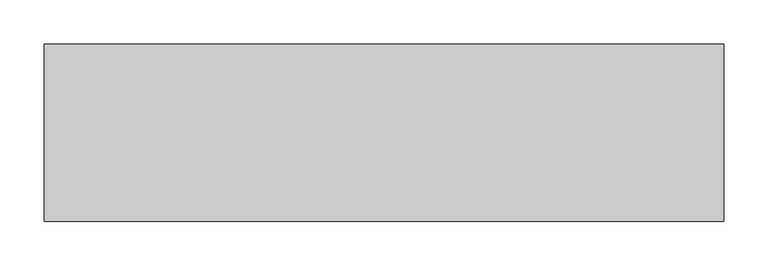
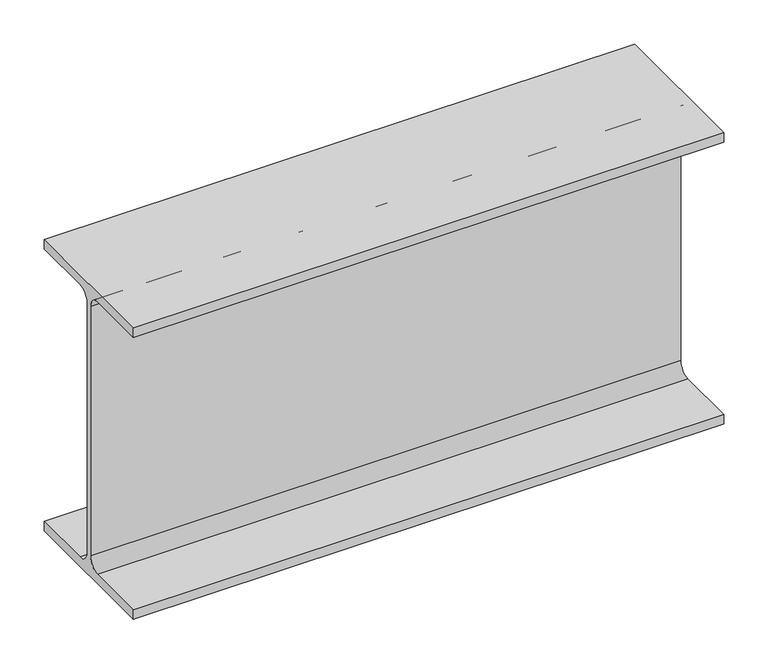
"""IFC4 building model written with IfcOpenShell, lengths in millimetres: beam geometry, Steel Framing_H_KS : H_SB_AR_S02_H-400x200x8x13_SCB1."""

from ifc_helpers import new_model, si_unit, point, frame, frame_2d, origin, place, context, project, spatial, polyline, circle_curve, trimmed, segment, composite_curve, outline, extrude, source, transform, mapped, element, save


def beam_d36fe593(model_context):
    return source(origin(), model_context, "Body", "SweptSolid", [
        extrude(outline(composite_curve([segment(polyline([(-100.0, -187.0), (-20.0, -187.0)]), True, "CONTINUOUS"), segment(trimmed(circle_curve(frame_2d((-20.0, -171.0)), 16.0), [point((-20.0, -187.0))], [point((-4.0, -171.0))], True, "CARTESIAN"), True, "CONTINUOUS"), segment(polyline([(-4.0, -171.0), (-4.0, 171.0)]), True, "CONTINUOUS"), segment(trimmed(circle_curve(frame_2d((-20.0, 171.0)), 16.0), [point((-4.0, 171.0))], [point((-20.0, 187.0))], True, "CARTESIAN"), True, "CONTINUOUS"), segment(polyline([(-20.0, 187.0), (-100.0, 187.0), (-100.0, 200.0), (100.0, 200.0), (100.0, 187.0), (20.0, 187.0)]), True, "CONTINUOUS"), segment(trimmed(circle_curve(frame_2d((20.0, 171.0)), 16.0), [point((20.0, 187.0))], [point((4.0, 171.0))], True, "CARTESIAN"), True, "CONTINUOUS"), segment(polyline([(4.0, 171.0), (4.0, -171.0)]), True, "CONTINUOUS"), segment(trimmed(circle_curve(frame_2d((20.0, -171.0)), 16.0), [point((4.0, -171.0))], [point((20.0, -187.0))], True, "CARTESIAN"), True, "CONTINUOUS"), segment(polyline([(20.0, -187.0), (100.0, -187.0), (100.0, -200.0), (-100.0, -200.0), (-100.0, -187.0)]), True, "CONTINUOUS")], self_intersect=False)), frame((-236.0, 0.0, 0.0), z_axis=(1.0, 0.0, 0.0), x_axis=(0.0, 1.0, 0.0)), (0.0, 0.0, 1.0), 766.0),
    ])


if __name__ == "__main__":
    model = new_model("IFC4")
    model_context = context("Model", 3, world=origin())
    ifc_project = project(units=[si_unit("LENGTHUNIT", "METRE", prefix="MILLI")], contexts=[model_context])
    site = spatial("IfcSite", under=ifc_project)
    building = spatial("IfcBuilding", under=site)
    placement = place(None, origin())
    beam_shape = beam_d36fe593(model_context)
    element("IfcBeam", 1, ObjectType="Steel Framing_H_KS : H_SB_AR_S02_H-400x200x8x13_SCB1", at=placement, inside=building, context=model_context, shape_type="MappedRepresentation", body=[
        mapped(beam_shape, transform((0.0, 0.0, 0.0), x_axis=(1.0, 0.0, 0.0), y_axis=(0.0, 1.0, 0.0), z_axis=(0.0, 0.0, 1.0))),
    ])
    save(model, "model.ifc")

# Revit data of these elements
# Type "Steel Framing_H_KS : H_SB_AR_S02_H-400x200x8x13_SCB1"
#   Type Comments = "MAIN"
#   Type Mark = "SCB1"
#   H_SectionID = "H-400x200x8x13"
#   H_Ratio for Additional Steel Plate = 0.2
#   Width = 20.0 cm
#   Web Thickness = 0.8 cm
#   Web Fillet = 1.6 cm
#   Warping Constant = 649000.0 cm⁶
#   Torsional Moment of Inertia = 35.8981 cm⁴
#   Section Area = 84.12 cm²
#   Plastic Modulus weak axis = 268.0 cm³
#   Plastic Modulus strong axis = 1330.0 cm³
#   Perimeter = 1.56 m²/m
#   Nominal Weight = 66.00 kgf/m
#   Moment of Inertia weak axis = 1740.00 cm⁴
#   Moment of Inertia strong axis = 23700.00 cm⁴
#   Height = 40.0 cm
#   Flange Thickness = 1.3 cm
#   Elastic Modulus weak axis = 174.0 cm³
#   Elastic Modulus strong axis = 1190.0 cm³
#   Centroid Vertical = 20.0 cm
#   Centroid Horizontal = 10.0 cm
#   Bolt Spacing = 8.89 cm
#   Length [instance default] = 1500 mm
#   Structural Material [instance default] = Steel, 45-345
#   Section Name Key = ""
#   Assembly Code = ""
# Element 1 (IfcBeam, "Steel Framing_H_KS : H_SB_AR_S02_H-400x200x8x13_SCB1")
#   Materials on its faces: "Steel, 45-345"
# Materials
#   "Steel, 45-345": class "Metal", colour RGB 189 187 185, transparency 0, Description = "Steel 345 MPa", Cost = 0
